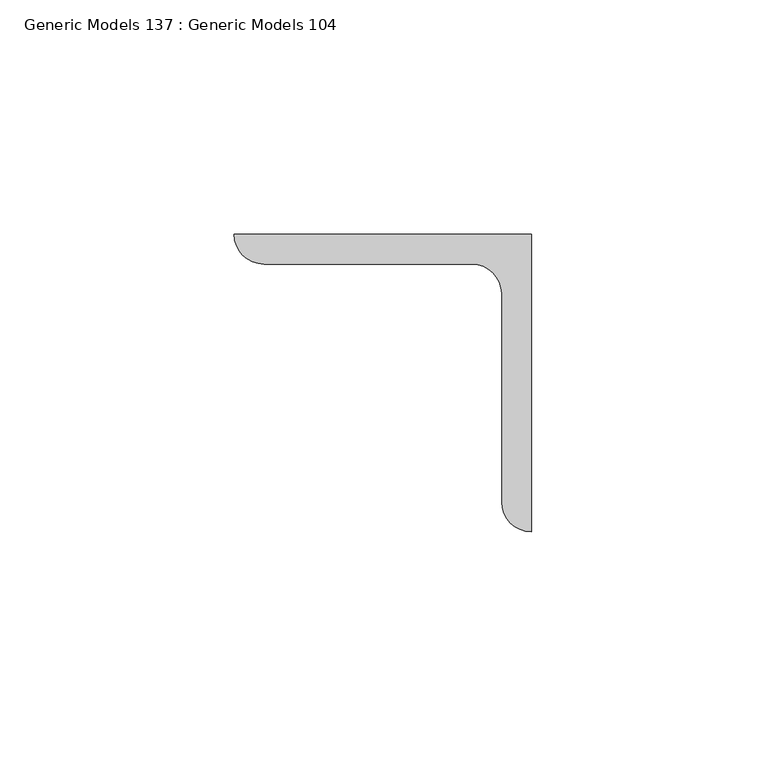
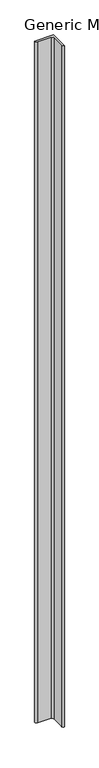
"""IFC4 building model written with IfcOpenShell, lengths in millimetres: proxy geometry, Generic Models 137 : Generic Models 104."""

from ifc_helpers import new_model, si_unit, point, frame, frame_2d, origin, place, context, project, spatial, polyline, circle_curve, trimmed, segment, composite_curve, outline, extrude, source, transform, mapped, element, save


def generic_models_137_generic_models_104_020ccf5d(model_context):
    return source(origin(), model_context, "Body", "SweptSolid", [
        extrude(outline(composite_curve([segment(polyline([(30226.3140778, 41071.1196612), (30226.3140778, 41007.6196612)]), True, "CONTINUOUS"), segment(trimmed(circle_curve(frame_2d((30226.3140778, 41013.9696612)), 6.35), [point((30226.3140778, 41007.6196612))], [point((30219.9640778, 41013.9696612))], False, "CARTESIAN"), True, "CONTINUOUS"), segment(polyline([(30219.9640778, 41013.9696612), (30219.9640778, 41058.4196612)]), True, "CONTINUOUS"), segment(trimmed(circle_curve(frame_2d((30213.6140778, 41058.4196612)), 6.35), [point((30219.9640778, 41058.4196612))], [point((30213.6140778, 41064.7696612))], True, "CARTESIAN"), True, "CONTINUOUS"), segment(polyline([(30213.6140778, 41064.7696612), (30169.1640778, 41064.7696612)]), True, "CONTINUOUS"), segment(trimmed(circle_curve(frame_2d((30169.1640778, 41071.1196612)), 6.35), [point((30169.1640778, 41064.7696612))], [point((30162.8140778, 41071.1196612))], False, "CARTESIAN"), True, "CONTINUOUS"), segment(polyline([(30162.8140778, 41071.1196612), (30226.3140778, 41071.1196612)]), True, "CONTINUOUS")], self_intersect=False)), frame((0.0, 0.0, 266407.9), z_axis=(0.0, 0.0, 1.0), x_axis=(1.0, 0.0, 0.0)), (0.0, 0.0, 1.0), 2432.1044757),
    ])


if __name__ == "__main__":
    model = new_model("IFC4")
    model_context = context("Model", 3, world=origin())
    ifc_project = project(units=[si_unit("LENGTHUNIT", "METRE", prefix="MILLI")], contexts=[model_context])
    site = spatial("IfcSite", under=ifc_project)
    building = spatial("IfcBuilding", under=site)
    placement = place(None, origin())
    generic_models_137_generic_models_104_shape = generic_models_137_generic_models_104_020ccf5d(model_context)
    element("IfcBuildingElementProxy", 1, Name="Generic Models 137 : Generic Models 104", ObjectType="Generic Models 137 : Generic Models 104", at=placement, inside=building, context=model_context, shape_type="MappedRepresentation", body=[
        mapped(generic_models_137_generic_models_104_shape, transform((0.0, 0.0, 0.0), x_axis=(1.0, 0.0, 0.0), y_axis=(0.0, 1.0, 0.0), z_axis=(0.0, 0.0, 1.0))),
    ])
    save(model, "model.ifc")

# Revit data of these elements
# Element 1 (IfcBuildingElementProxy, "Generic Models 137 : Generic Models 104")
#   Materials on its faces: "(2) BACK/BACK GALVANIZED ANGLES (2) L2 1/2 X 2 1/2 X 1/4\")"
# Materials
#   "(2) BACK/BACK GALVANIZED ANGLES (2) L2 1/2 X 2 1/2 X 1/4\")": class "Unassigned", colour RGB 211 211 211, transparency 0, Cost = 0
